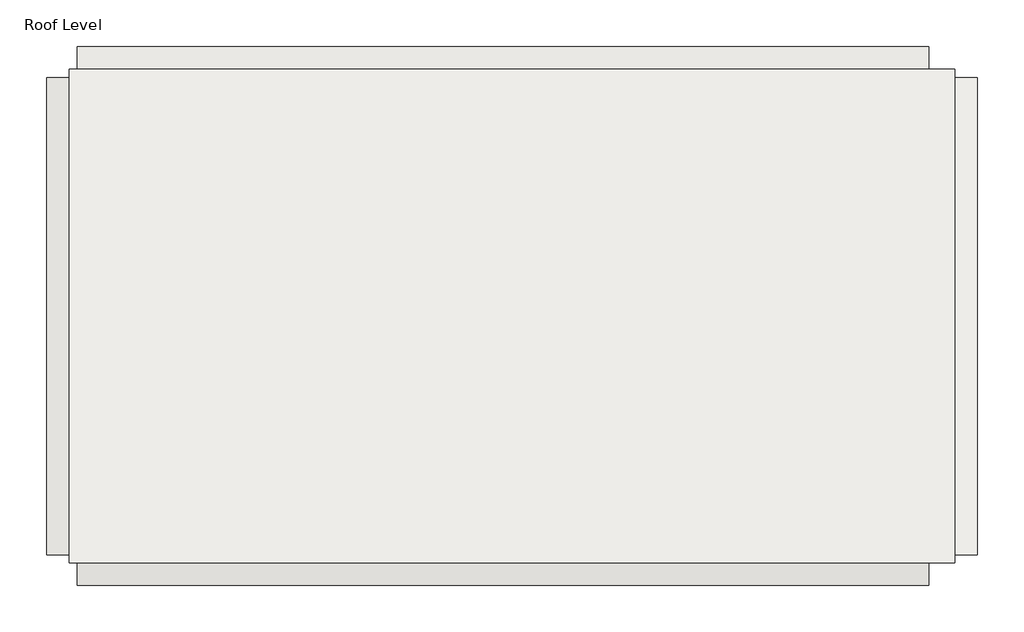
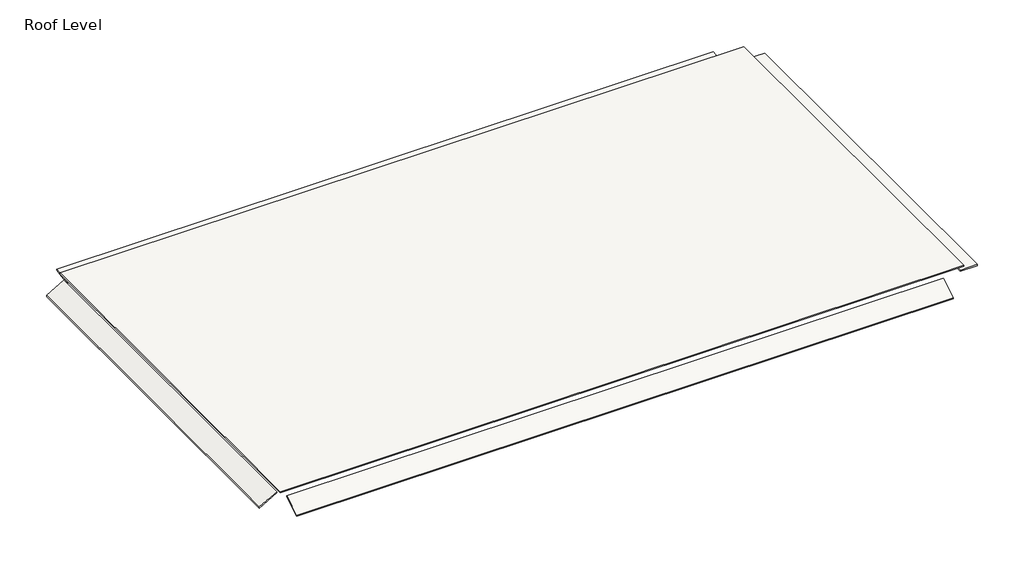
# One storey: 5 roofs.
"""IFC4 building model written with IfcOpenShell, lengths in millimetres."""

import ifcopenshell
import ifcopenshell.guid

model = None  # the IFC model being written
_history = None  # IfcOwnerHistory: only IFC2X3 demands one
_inside = {}  # id of a spatial element -> (the spatial element, [elements in it])
_under = {}  # id of a project, library or spatial element -> (it, [spatial elements below it])
_declared = {}  # id of a project -> (the project, [libraries it declares])
_typed = {}  # id of a type object -> (the type object, [elements of that type])
_made_of = {}  # id of a material, layer set ... -> (it, [elements and type objects made of it])


def new_model(schema):
    """Start an empty IFC model of exactly this schema.

    Asked for "IFC4X3", IfcOpenShell would pick the latest addendum, in which some entities
    have other attributes; the version numbers below select the first issue.
    IFC2X3 requires an IfcOwnerHistory on every rooted entity: one is made here for all.
    """
    global model, _history
    if schema == "IFC4X3":
        model = ifcopenshell.file(schema_version=(4, 3, 0, 0))
    else:
        model = ifcopenshell.file(schema=schema)
    _inside.clear()
    _under.clear()
    _declared.clear()
    _typed.clear()
    _made_of.clear()
    _history = None
    if model.schema == "IFC2X3":
        org = make("IfcOrganization", Name="unknown")
        user = make(
            "IfcPersonAndOrganization",
            ThePerson=make("IfcPerson", FamilyName="unknown"),
            TheOrganization=org,
        )
        app = make(
            "IfcApplication",
            ApplicationDeveloper=org,
            Version="unknown",
            ApplicationFullName="unknown",
            ApplicationIdentifier="unknown",
        )
        _history = make(
            "IfcOwnerHistory",
            OwningUser=user,
            OwningApplication=app,
            ChangeAction="ADDED",
            CreationDate=0,
        )
    return model


def make(cls, **values):
    """One entity of the class cls with the attributes given. An attribute that is None is left unset."""
    return model.create_entity(
        cls, **{name: value for name, value in values.items() if value is not None}
    )


def rooted(cls, **values):
    """An entity with a GlobalId (a new one), such as an element, a storey or a relation."""
    return make(cls, GlobalId=ifcopenshell.guid.new(), OwnerHistory=_history, **values)


def si_unit(unit_type, name, prefix=None):
    """IfcSIUnit, for example si_unit("LENGTHUNIT", "METRE", prefix="MILLI")."""
    return make("IfcSIUnit", UnitType=unit_type, Prefix=prefix, Name=name)


def assignment(units):
    """IfcUnitAssignment: the units of a project."""
    return None if units is None else make("IfcUnitAssignment", Units=units)


def point(xyz):
    """IfcCartesianPoint."""
    return None if xyz is None else make("IfcCartesianPoint", Coordinates=xyz)


def direction(xyz):
    """IfcDirection."""
    return None if xyz is None else make("IfcDirection", DirectionRatios=xyz)


def frame(location, z_axis=None, x_axis=None):
    """IfcAxis2Placement3D, a coordinate frame: its origin and axes. An axis left out is left unset."""
    return make(
        "IfcAxis2Placement3D",
        Location=point(location),
        Axis=direction(z_axis),
        RefDirection=direction(x_axis),
    )


def origin():
    """The frame at (0, 0, 0) with its axes left unset."""
    return frame((0.0, 0.0, 0.0))


def place(relative_to, where):
    """IfcLocalPlacement: puts the frame where relative to a parent placement (None: the world)."""
    return make(
        "IfcLocalPlacement", PlacementRelTo=relative_to, RelativePlacement=where
    )


def context(
    kind, dimensions, precision=None, world=None, true_north=None, identifier=None
):
    """IfcGeometricRepresentationContext, for example the 3D "Model" context."""
    return make(
        "IfcGeometricRepresentationContext",
        ContextIdentifier=identifier,
        ContextType=kind,
        CoordinateSpaceDimension=dimensions,
        Precision=precision,
        WorldCoordinateSystem=world,
        TrueNorth=true_north,
    )


def project(units=None, contexts=None):
    """IfcProject with its units and contexts."""
    return rooted(
        "IfcProject",
        Name="project",
        RepresentationContexts=contexts,
        UnitsInContext=assignment(units),
    )


def spatial(cls, under=None, at=None, **own):
    """A site, building, storey or space (cls), placed at a placement, below another one or the project."""
    s = rooted(cls, ObjectPlacement=at, **own)
    if under is not None:
        _under.setdefault(under.id(), (under, []))[1].append(s)
    return s


def polyline(points):
    """IfcPolyline through the points."""
    return make("IfcPolyline", Points=[point(p) for p in points])


def outline(outer, holes=None, kind="AREA"):
    """IfcArbitraryClosedProfileDef: a profile drawn as a closed curve; with holes, ...WithVoids."""
    if holes is None:
        return make("IfcArbitraryClosedProfileDef", ProfileType=kind, OuterCurve=outer)
    return make(
        "IfcArbitraryProfileDefWithVoids",
        ProfileType=kind,
        OuterCurve=outer,
        InnerCurves=holes,
    )


def extrude(swept, where, along, depth):
    """IfcExtrudedAreaSolid: the profile swept, set in the frame where, extruded along a direction by depth."""
    return make(
        "IfcExtrudedAreaSolid",
        SweptArea=swept,
        Position=where,
        ExtrudedDirection=direction(along),
        Depth=depth,
    )


def shape(context_of_items, identifier, shape_type, items):
    """IfcShapeRepresentation: the items that make up one representation, for example the "Body"."""
    return make(
        "IfcShapeRepresentation",
        ContextOfItems=context_of_items,
        RepresentationIdentifier=identifier,
        RepresentationType=shape_type,
        Items=items,
    )


def made_of(thing, what):
    """Note that an element or type object is made of a material, layer set ...; save() writes the relation."""
    if what is not None:
        _made_of.setdefault(what.id(), (what, []))[1].append(thing)
    return thing


def element(
    cls,
    number,
    at=None,
    inside=None,
    cuts=None,
    type_object=None,
    material=None,
    context=None,
    identifier="Body",
    shape_type=None,
    held_by="IfcProductDefinitionShape",
    body=None,
    shapes=None,
    **own,
):
    """One element of the class cls, such as IfcWall. Its Tag is "e" and its number.

    at: its placement. inside: the storey or other place that contains it. cuts: it is an
    opening in that element (IfcRelVoidsElement). A single representation is given by context,
    identifier, shape_type and body (its items); several are given by shapes. held_by: the class
    of the entity that holds the representations. save() writes the other relations.
    """
    e = rooted(cls, Tag="e%d" % number, ObjectPlacement=at, **own)
    if body is not None:
        shapes = [shape(context, identifier, shape_type, body)]
    if shapes is not None:
        e.Representation = make(held_by, Representations=shapes)
    if inside is not None:
        _inside.setdefault(inside.id(), (inside, []))[1].append(e)
    if cuts is not None:
        rooted(
            "IfcRelVoidsElement", RelatingBuildingElement=cuts, RelatedOpeningElement=e
        )
    if type_object is not None:
        _typed.setdefault(type_object.id(), (type_object, []))[1].append(e)
    return made_of(e, material)


def aggregate(whole, parts):
    """IfcRelAggregates: a whole, such as a stair, and the parts it consists of."""
    return rooted("IfcRelAggregates", RelatingObject=whole, RelatedObjects=parts)


def save(model, path):
    """Write the relations noted so far, then the file.

    IfcRelAggregates (storeys below a building ...), IfcRelContainedInSpatialStructure (elements
    in a storey), IfcRelDefinesByType, IfcRelAssociatesMaterial and IfcRelDeclares: one each for
    every whole, place, type object, material and project.
    """
    for whole, parts in _under.values():
        aggregate(whole, parts)
    for where, things in _inside.values():
        rooted(
            "IfcRelContainedInSpatialStructure",
            RelatedElements=things,
            RelatingStructure=where,
        )
    for kind, things in _typed.values():
        rooted("IfcRelDefinesByType", RelatedObjects=things, RelatingType=kind)
    for what, things in _made_of.values():
        rooted("IfcRelAssociatesMaterial", RelatedObjects=things, RelatingMaterial=what)
    for by, libraries in _declared.values():
        rooted("IfcRelDeclares", RelatingContext=by, RelatedDefinitions=libraries)
    model.write(path)


model = new_model("IFC4")

# Units and contexts
model_context = context("Model", 3, world=origin())
ifc_project = project(units=[si_unit("LENGTHUNIT", "METRE", prefix="MILLI")], contexts=[model_context])

# Site, building, storey
site = spatial("IfcSite", under=ifc_project)
building = spatial("IfcBuilding", under=site)
storey = spatial("IfcBuildingStorey", under=building, Name="Roof Level", Elevation=7924.8)

# Roofs
placement = place(None, origin())
element("IfcRoof", 1, ObjectType="Shading devices - 50mm", at=placement, inside=storey, context=model_context, shape_type="SweptSolid", body=[
    extrude(outline(polyline([(-4795.4197783, 7308.2548116), (-4095.4197783, 7712.4), (-4095.4197783, 7654.6649731), (-4795.4197783, 7250.5197846), (-4795.4197783, 7308.2548116)])), frame((1746.464681, 0.0, 0.0), z_axis=(1.0, 0.0, 0.0), x_axis=(0.0, 1.0, 0.0)), (0.0, 0.0, 1.0), 26500.0),
])
element("IfcRoof", 2, ObjectType="Shading devices - 50mm", at=placement, inside=storey, context=model_context, shape_type="SweptSolid", body=[
    extrude(outline(polyline([(29068.464681, 11030.5802217), (29768.464681, 11030.5802217), (29768.464681, -3843.0197783), (29068.464681, -3843.0197783), (29068.464681, 11030.5802217)])), frame((0.0, 0.0, 7562.4), z_axis=(0.0, 0.0, 1.0), x_axis=(1.0, 0.0, 0.0)), (0.0, 0.0, 1.0), 50.0),
])
element("IfcRoof", 3, ObjectType="Shading devices - 50mm", at=placement, inside=storey, context=model_context, shape_type="SweptSolid", body=[
    extrude(outline(polyline([(11296.9802217, 7489.7424441), (11996.9802217, 7613.1713306), (11996.9802217, 7562.4), (11296.9802217, 7438.9711135), (11296.9802217, 7489.7424441)])), frame((1746.464681, 0.0, 0.0), z_axis=(1.0, 0.0, 0.0), x_axis=(0.0, 1.0, 0.0)), (0.0, 0.0, 1.0), 26500.0),
])
element("IfcRoof", 4, ObjectType="Shading devices - 50mm", at=placement, inside=storey, context=model_context, shape_type="SweptSolid", body=[
    extrude(outline(polyline([(7824.8, 1484.064681), (7420.6548116, 784.064681), (7362.9197846, 784.064681), (7767.0649731, 1484.064681), (7824.8, 1484.064681)])), frame((0.0, -3843.0197783, 0.0), z_axis=(0.0, 1.0, 0.0), x_axis=(0.0, 0.0, 1.0)), (0.0, 0.0, 1.0), 14873.6),
])
element("IfcRoof", 5, ObjectType="Shading devices - 50mm", at=placement, inside=storey, context=model_context, shape_type="SweptSolid", body=[
    extrude(outline(polyline([(1484.064681, 11296.9802217), (29068.464681, 11296.9802217), (29068.464681, -4095.4197783), (1484.064681, -4095.4197783), (1484.064681, 11296.9802217)])), frame((0.0, 0.0, 7924.8), z_axis=(0.0, 0.0, 1.0), x_axis=(1.0, 0.0, 0.0)), (0.0, 0.0, 1.0), 50.0),
])

save(model, "model.ifc")

# Revit data of these elements
# Type "Shading devices - 50mm"
#   Layers, outside or top first: 50 mm no material (function 1)
# Element 1 (IfcRoof, "Shading devices - 50mm")
#   built-in parameter 1001705 = 25.3031 (stored number, unit not read)
#   built-in parameter 1001701 = -2.21221 (stored number, unit not read)
#   built-in parameter 1001710 = 33615
#   Phase Created = New Construction
#   Materials on its faces: "Default Roof"
# Element 2 (IfcRoof, "Shading devices - 50mm")
#   built-in parameter 1001705 = 24.9751 (stored number, unit not read)
#   built-in parameter 1001701 = -1.18898 (stored number, unit not read)
#   built-in parameter 1001710 = 33615
#   Phase Created = New Construction
#   Materials on its faces: "Default Roof"
# Element 3 (IfcRoof, "Shading devices - 50mm")
#   built-in parameter 1001705 = 24.9776 (stored number, unit not read)
#   built-in parameter 1001701 = -1.18898 (stored number, unit not read)
#   built-in parameter 1001710 = 33615
#   Phase Created = New Construction
#   Materials on its faces: "Default Roof"
# Element 4 (IfcRoof, "Shading devices - 50mm")
#   built-in parameter 1001705 = 25.6719 (stored number, unit not read)
#   built-in parameter 1001701 = -1.84344 (stored number, unit not read)
#   built-in parameter 1001710 = 33615
#   Phase Created = New Construction
#   Materials on its faces: "Default Roof"
# Element 5 (IfcRoof, "Shading devices - 50mm")
#   built-in parameter 1001705 = 26.164 (stored number, unit not read)
#   built-in parameter 1001710 = 33615
#   Phase Created = New Construction
#   Materials on its faces: "Default Roof"
# Materials
#   "Default Roof": class "Miscellaneous", colour RGB 0 127 0, transparency 0, Cost = 0
